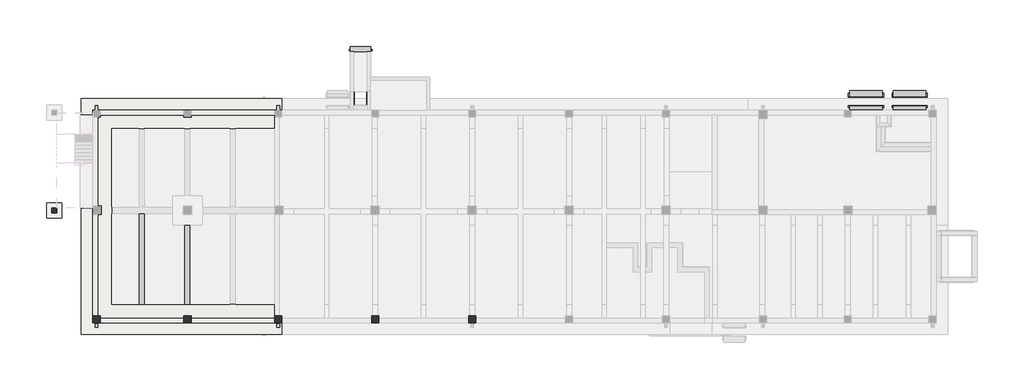
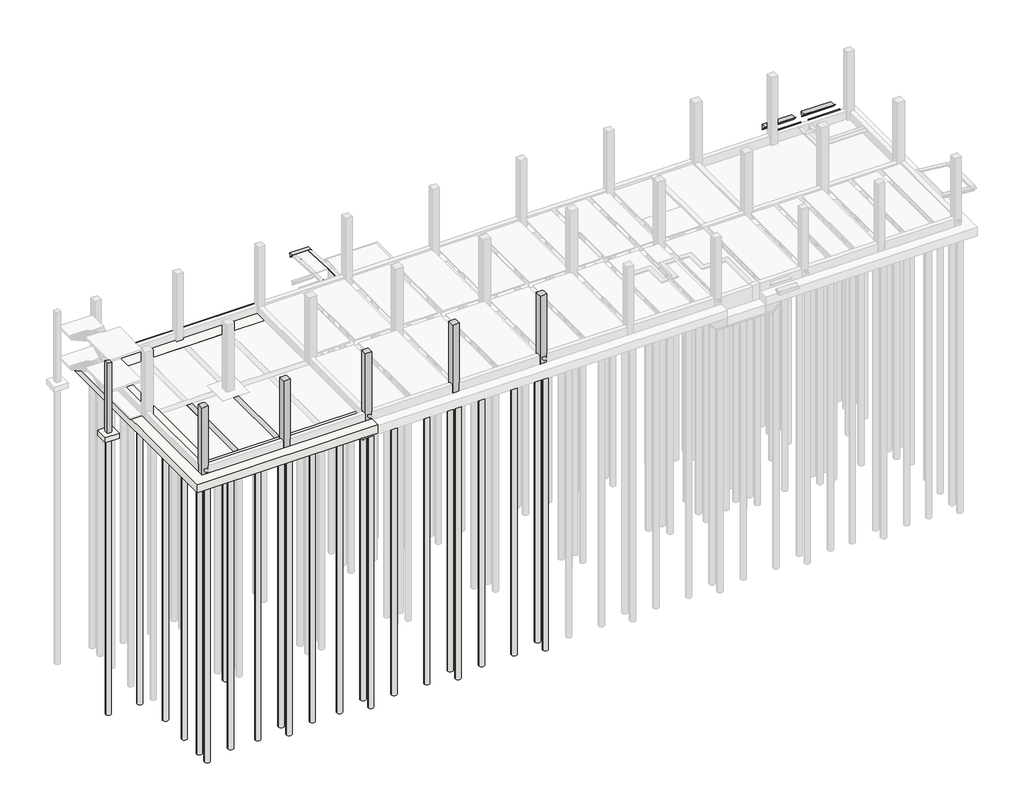
# One storey, part 3 of 7: 26 slabs, 11 proxies, 6 columns, 2 beams.
"""IFC4 building model written with IfcOpenShell, lengths in millimetres."""

from ifc_helpers import new_model, si_unit, point, frame, frame_2d, origin, place, context, project, spatial, polyline, circle_curve, trimmed, segment, composite_curve, outline, extrude, faceted_brep, element, save

model = new_model("IFC4")

# Units and contexts
model_context = context("Model", 3, world=origin())
ifc_project = project(units=[si_unit("LENGTHUNIT", "METRE", prefix="MILLI")], contexts=[model_context])

# Site, building, storey
site = spatial("IfcSite", under=ifc_project)
building = spatial("IfcBuilding", under=site)
storey = spatial("IfcBuildingStorey", under=building, Name="H.P.P", Elevation=4500.0)

# Beams
placement = place(None, origin())
element("IfcBeam", 1, ObjectType="RC Beam_Rectangular : H_SB_AR S16_TG-UG_500x700_FB1A", at=placement, inside=storey, context=model_context, shape_type="Brep", body=[
    faceted_brep([(3500.0, -15750.0, 3400.0), (4000.0, -15750.0, 3400.0), (4000.0, -15750.0, 3840.0), (4000.0, -15750.0, 3950.0), (4000.0, -15750.0, 4100.0), (3500.0, -15750.0, 4100.0), (3500.0, -15750.0, 3950.0), (3500.0, -15750.0, 3840.0), (4000.0, -8300.0, 4100.0), (3500.0, -8300.0, 4100.0), (4000.0, -8300.0, 3950.0), (4000.0, -8300.0, 3400.0), (4000.0, -8300.0, 3840.0), (3500.0, -8300.0, 3400.0), (3500.0, -8300.0, 3950.0), (3500.0, -8300.0, 3840.0)], [[[0, 1, 2, 3, 4, 5, 6, 7]], [[5, 4, 8, 9]], [[10, 8, 4, 3, 2, 1, 11, 12]], [[1, 0, 13, 11]], [[9, 14, 15, 13, 0, 7, 6, 5]], [[9, 8, 10, 12, 11, 13, 15, 14]]]),
])
element("IfcBeam", 2, ObjectType="RC Beam_Rectangular : H_SB_AR S16_TG-UG_500x700_FG1", at=placement, inside=storey, context=model_context, shape_type="Brep", body=[
    faceted_brep([(7250.0, -9250.0, 4100.0), (7750.0, -9250.0, 4100.0), (7750.0, -9250.0, 3950.0), (7750.0, -9250.0, 3840.0), (7750.0, -9250.0, 3400.0), (7250.0, -9250.0, 3400.0), (7250.0, -9250.0, 3840.0), (7250.0, -9250.0, 3950.0), (7250.0, -15750.0, 3400.0), (7750.0, -15750.0, 3400.0), (7750.0, -15750.0, 3840.0), (7750.0, -15750.0, 3950.0), (7750.0, -15750.0, 4100.0), (7250.0, -15750.0, 4100.0), (7250.0, -15750.0, 3950.0), (7250.0, -15750.0, 3840.0)], [[[0, 1, 2, 3, 4, 5, 6, 7]], [[8, 9, 10, 11, 12, 13, 14, 15]], [[1, 0, 13, 12]], [[1, 12, 11, 10, 9, 4, 3, 2]], [[5, 4, 9, 8]], [[13, 0, 7, 6, 5, 8, 15, 14]]]),
])

# Proxies
element("IfcBuildingElementProxy", 3, Name="H_SF_AR_B08_Stoop_T150_FrontEdge", ObjectType="H_SF_AR_B08_Stoop_T150_FrontEdge", at=placement, inside=storey, context=model_context, shape_type="SweptSolid", body=[
    extrude(outline(polyline([(312.0000074, 4450.0), (312.0000074, 4600.0), (662.0000074, 4600.0), (512.0000074, 4450.0), (312.0000074, 4450.0)])), frame((65750.0, 0.0, 0.0), z_axis=(1.0, 0.0, 0.0), x_axis=(0.0, 1.0, 0.0)), (0.0, 0.0, 1.0), 2700.0),
])
element("IfcBuildingElementProxy", 4, Name="H_SF_AR_B08_Stoop_T150_FrontEdge_500x300", ObjectType="H_SF_AR_B08_Stoop_T150_FrontEdge_500x300", at=placement, inside=storey, context=model_context, shape_type="Brep", body=[
    faceted_brep([(68450.0, 1900.0, 4300.0), (68450.0, 1900.0, 4600.0), (68450.0, 1600.0, 4600.0), (68450.0, 1400.0, 4600.0), (68450.0, 1700.0, 4300.0), (65750.0, 1900.0, 4300.0), (65750.0, 1700.0, 4300.0), (65750.0, 1400.0, 4600.0), (65750.0, 1600.0, 4600.0), (65750.0, 1900.0, 4600.0)], [[[0, 1, 2, 3, 4]], [[5, 6, 7, 8, 9]], [[1, 0, 5, 9]], [[3, 2, 1, 9, 8, 7]], [[4, 3, 7, 6]], [[0, 4, 6, 5]]]),
])
element("IfcBuildingElementProxy", 5, Name="H_SF_AR_S18_Lean_T50_300X300", ObjectType="H_SF_AR_S18_Lean_T50_300X300", at=placement, inside=storey, context=model_context, shape_type="SweptSolid", body=[
    extrude(outline(polyline([(1700.0, 4300.0), (1700.0, 4250.0), (1679.2893219, 4250.0), (1379.2893219, 4550.0), (1400.0, 4550.0), (1400.0, 4600.0), (1700.0, 4300.0)])), frame((65650.0, 0.0, 0.0), z_axis=(1.0, 0.0, 0.0), x_axis=(0.0, 1.0, 0.0)), (0.0, 0.0, 1.0), 2900.0),
])
element("IfcBuildingElementProxy", 6, Name="H_SF_AR_S18_Lean_T50_150X150", ObjectType="H_SF_AR_S18_Lean_T50_150X150", at=placement, inside=storey, context=model_context, shape_type="SweptSolid", body=[
    extrude(outline(polyline([(512.0000074, 4400.0), (512.0000074, 4450.0), (662.0000074, 4600.0), (662.0000074, 4550.0), (682.7106855, 4550.0), (532.7106855, 4400.0), (512.0000074, 4400.0)])), frame((65650.0, 0.0, 0.0), z_axis=(1.0, 0.0, 0.0), x_axis=(0.0, 1.0, 0.0)), (0.0, 0.0, 1.0), 2900.0),
])
element("IfcBuildingElementProxy", 7, Name="H_SF_AR_B08_Stoop_T150_FrontEdge", ObjectType="H_SF_AR_B08_Stoop_T150_FrontEdge", at=placement, inside=storey, context=model_context, shape_type="SweptSolid", body=[
    extrude(outline(polyline([(312.0000074, 4450.0), (312.0000074, 4600.0), (662.0000074, 4600.0), (512.0000074, 4450.0), (312.0000074, 4450.0)])), frame((62150.0, 0.0, 0.0), z_axis=(1.0, 0.0, 0.0), x_axis=(0.0, 1.0, 0.0)), (0.0, 0.0, 1.0), 2700.0),
])
element("IfcBuildingElementProxy", 8, Name="H_SF_AR_B08_Stoop_T150_FrontEdge_500x300", ObjectType="H_SF_AR_B08_Stoop_T150_FrontEdge_500x300", at=placement, inside=storey, context=model_context, shape_type="Brep", body=[
    faceted_brep([(64850.0, 1900.0, 4300.0), (64850.0, 1900.0, 4600.0), (64850.0, 1600.0, 4600.0), (64850.0, 1400.0, 4600.0), (64850.0, 1700.0, 4300.0), (62150.0, 1900.0, 4300.0), (62150.0, 1700.0, 4300.0), (62150.0, 1400.0, 4600.0), (62150.0, 1600.0, 4600.0), (62150.0, 1900.0, 4600.0)], [[[0, 1, 2, 3, 4]], [[5, 6, 7, 8, 9]], [[1, 0, 5, 9]], [[3, 2, 1, 9, 8, 7]], [[4, 3, 7, 6]], [[0, 4, 6, 5]]]),
])
element("IfcBuildingElementProxy", 9, Name="H_SF_AR_S18_Lean_T50_300X300", ObjectType="H_SF_AR_S18_Lean_T50_300X300", at=placement, inside=storey, context=model_context, shape_type="SweptSolid", body=[
    extrude(outline(polyline([(1700.0, 4300.0), (1700.0, 4250.0), (1679.2893219, 4250.0), (1379.2893219, 4550.0), (1400.0, 4550.0), (1400.0, 4600.0), (1700.0, 4300.0)])), frame((62050.0, 0.0, 0.0), z_axis=(1.0, 0.0, 0.0), x_axis=(0.0, 1.0, 0.0)), (0.0, 0.0, 1.0), 2900.0),
])
element("IfcBuildingElementProxy", 10, Name="H_SF_AR_S18_Lean_T50_150X150", ObjectType="H_SF_AR_S18_Lean_T50_150X150", at=placement, inside=storey, context=model_context, shape_type="SweptSolid", body=[
    extrude(outline(polyline([(512.0000074, 4400.0), (512.0000074, 4450.0), (662.0000074, 4600.0), (662.0000074, 4550.0), (682.7106855, 4550.0), (532.7106855, 4400.0), (512.0000074, 4400.0)])), frame((62050.0, 0.0, 0.0), z_axis=(1.0, 0.0, 0.0), x_axis=(0.0, 1.0, 0.0)), (0.0, 0.0, 1.0), 2900.0),
])
element("IfcBuildingElementProxy", 11, Name="H_SF_AR_B08_Ramp_T150_FrontEdge(SLOPE)", ObjectType="H_SF_AR_B08_Ramp_T150_FrontEdge(SLOPE)", at=placement, inside=storey, context=model_context, shape_type="Brep", body=[
    faceted_brep([(22638.0, 5300.0, 4179.6670362), (22638.0, 5550.0, 4179.6670362), (22638.0, 5550.0, 4349.6670362), (22638.0, 5100.0, 4379.6670362), (22638.0, 5261.0710326, 4218.5960036), (20938.0, 5550.0, 4179.6670362), (20938.0, 5300.0, 4179.6670362), (20938.0, 5261.0710326, 4218.5960036), (20938.0, 5100.0, 4379.6670362), (20938.0, 5550.0, 4349.6670362), (22338.0, 5100.0, 4379.6670362), (21238.0, 5100.0, 4379.6670362)], [[[0, 1, 2, 3, 4]], [[5, 6, 7, 8, 9]], [[1, 5, 9, 2]], [[1, 0, 6, 5]], [[0, 4, 3, 10, 11, 8, 7, 6]], [[3, 2, 9, 8, 11, 10]]]),
])
element("IfcBuildingElementProxy", 12, Name="H_SF_AR_S18_Lean_T50_200X200", ObjectType="H_SF_AR_S18_Lean_T50_200X200", at=placement, inside=storey, context=model_context, shape_type="Brep", body=[
    faceted_brep([(20838.0, 5300.0, 4179.6670362), (20838.0, 5300.0, 4129.6670362), (20838.0, 5279.2893219, 4129.6670362), (20838.0, 5184.596098, 4224.3602601), (20838.0, 5260.3575388, 4219.3094974), (22738.0, 5300.0, 4129.6670362), (22738.0, 5300.0, 4179.6670362), (22738.0, 5260.3575388, 4219.3094974), (22738.0, 5184.596098, 4224.3602601), (22738.0, 5238.2864422, 4170.6699159), (22738.0, 5279.2893219, 4129.6670362), (20938.0, 5260.3575388, 4219.3094974), (20938.0, 5261.0710326, 4218.5960036), (21088.0, 5261.0710326, 4218.5960036), (21238.0, 5100.0, 4379.6670362), (22338.0, 5100.0, 4379.6670362), (22488.0, 5261.0710326, 4218.5960036), (22638.0, 5261.0710326, 4218.5960036), (22638.0, 5260.3575388, 4219.3094974), (22638.0, 5300.0, 4179.6670362), (20938.0, 5300.0, 4179.6670362), (22638.0, 5184.596098, 4224.3602601), (22638.0, 5185.3095918, 4223.6467663), (22488.0, 5185.3095918, 4223.6467663), (22389.2669117, 5079.2893219, 4329.6670362), (22319.2206862, 5079.2893219, 4329.6670362), (21256.7793138, 5079.2893219, 4329.6670362), (21186.7330883, 5079.2893219, 4329.6670362), (21088.0, 5185.3095918, 4223.6467663), (20938.0, 5185.3095918, 4223.6467663), (20938.0, 5184.596098, 4224.3602601), (20850.0, 5184.596098, 4224.3602601), (22387.8892579, 5100.0, 4329.6670362), (22317.8430324, 5100.0, 4329.6670362), (21258.1569676, 5100.0, 4329.6670362), (21188.1107421, 5100.0, 4329.6670362)], [[[0, 1, 2, 3, 4]], [[5, 6, 7, 8, 9, 10]], [[0, 4, 11, 12, 13, 14, 15, 16, 17, 18, 7, 6, 19, 20]], [[1, 0, 20, 19, 6, 5]], [[2, 1, 5, 10]], [[2, 10, 9, 8, 21, 22, 23, 24, 25, 26, 27, 28, 29, 30, 31, 3]], [[27, 26, 25, 24, 32, 33, 34, 35]], [[15, 14, 35, 34, 33, 32]], [[8, 7, 18, 21]], [[4, 3, 31, 30, 11]], [[29, 12, 11, 30]], [[13, 28, 27, 35, 14]], [[12, 29, 28, 13]], [[17, 22, 21, 18]], [[23, 16, 15, 32, 24]], [[22, 17, 16, 23]]]),
])
element("IfcBuildingElementProxy", 13, Name="H_SF_AR_S18_Lean_T50_150X150", ObjectType="H_SF_AR_S18_Lean_T50_150X150", at=placement, inside=storey, context=model_context, shape_type="Brep", body=[
    faceted_brep([(22338.0, 1800.0, 4600.0), (22488.0, 1800.0, 4450.0), (22488.0, 1800.0, 4400.0), (22467.2893219, 1800.0, 4400.0), (22317.2893219, 1800.0, 4550.0), (22338.0, 1800.0, 4550.0), (22488.0, 550.0, 4450.0), (22338.0, 700.0, 4600.0), (22338.0, 700.0, 4550.0), (22317.2893219, 720.7106781, 4550.0), (22467.2893219, 570.7106781, 4400.0), (22488.0, 550.0, 4400.0)], [[[0, 1, 2, 3, 4, 5]], [[6, 7, 8, 9, 10, 11]], [[1, 0, 7, 6]], [[2, 1, 6, 11]], [[3, 2, 11, 10]], [[4, 3, 10, 9]], [[5, 4, 9, 8]], [[0, 5, 8, 7]]]),
    faceted_brep([(21238.0, 700.0, 4600.0), (21088.0, 550.0, 4450.0), (21088.0, 550.0, 4400.0), (21108.7106781, 570.7106781, 4400.0), (21258.7106781, 720.7106781, 4550.0), (21238.0, 700.0, 4550.0), (21088.0, 1800.0, 4450.0), (21238.0, 1800.0, 4600.0), (21238.0, 1800.0, 4550.0), (21258.7106781, 1800.0, 4550.0), (21108.7106781, 1800.0, 4400.0), (21088.0, 1800.0, 4400.0)], [[[0, 1, 2, 3, 4, 5]], [[6, 7, 8, 9, 10, 11]], [[1, 0, 7, 6]], [[2, 1, 6, 11]], [[3, 2, 11, 10]], [[4, 3, 10, 9]], [[5, 4, 9, 8]], [[0, 5, 8, 7]]]),
    faceted_brep([(22488.0, 1800.0, 4450.0), (22338.0, 1800.0, 4600.3329638), (22338.0, 1800.0, 4550.2219759), (22317.2893219, 1800.0, 4550.2219759), (22467.2893219, 1800.0, 4399.8890121), (22488.0, 1800.0, 4399.8890121), (22488.0, 5184.596098, 4224.3602601), (22389.9313644, 5079.2893219, 4329.6670362), (22388.5537105, 5100.0, 4329.6670362), (22338.6644526, 5100.0, 4379.6670362), (22338.0, 5109.9889135, 4379.6670362), (22488.0, 5238.2864422, 4170.6699159), (22467.2893219, 5238.2864422, 4170.6699159), (22317.2893219, 5100.0, 4330.2219759), (22317.8430324, 5100.0, 4329.6670362), (22319.2206862, 5079.2893219, 4329.6670362), (22338.0, 5100.0, 4330.2219759), (22338.0, 5100.0, 4379.6670362), (22389.2669117, 5079.2893219, 4329.6670362), (22387.8892579, 5100.0, 4329.6670362)], [[[0, 1, 2, 3, 4, 5]], [[1, 0, 6, 7, 8, 9, 10]], [[0, 5, 11, 6]], [[5, 4, 12, 11]], [[4, 3, 13, 14, 15, 12]], [[3, 2, 16, 13]], [[2, 1, 10, 17, 16]], [[10, 9, 17]], [[15, 18, 7, 6, 11, 12]], [[7, 18, 15, 14, 19, 8]], [[8, 19, 14, 13, 16, 17, 9]]]),
    faceted_brep([(21238.0, 1800.0, 4600.3329638), (21088.0, 1800.0, 4450.0), (21088.0, 1800.0, 4399.8890121), (21108.7106781, 1800.0, 4399.8890121), (21258.7106781, 1800.0, 4550.2219759), (21238.0, 1800.0, 4550.2219759), (21238.0, 5109.9889135, 4379.6670362), (21237.3355474, 5100.0, 4379.6670362), (21187.4462895, 5100.0, 4329.6670362), (21186.0686356, 5079.2893219, 4329.6670362), (21088.0, 5184.596098, 4224.3602601), (21088.0, 5238.2864422, 4170.6699159), (21108.7106781, 5238.2864422, 4170.6699159), (21256.7793138, 5079.2893219, 4329.6670362), (21258.1569676, 5100.0, 4329.6670362), (21258.7106781, 5100.0, 4330.2219759), (21238.0, 5100.0, 4330.2219759), (21238.0, 5100.0, 4379.6670362), (21186.7330883, 5079.2893219, 4329.6670362), (21188.1107421, 5100.0, 4329.6670362)], [[[0, 1, 2, 3, 4, 5]], [[1, 0, 6, 7, 8, 9, 10]], [[2, 1, 10, 11]], [[3, 2, 11, 12]], [[4, 3, 12, 13, 14, 15]], [[5, 4, 15, 16]], [[0, 5, 16, 17, 6]], [[7, 6, 17]], [[9, 18, 13, 12, 11, 10]], [[13, 18, 9, 8, 19, 14]], [[14, 19, 8, 7, 17, 16, 15]]]),
])

# Columns
element("IfcColumn", 14, ObjectType="RC_Column_Rectangular : H_SC_AR S15_RC Col-AG_600x600_C2", at=placement, inside=storey, context=model_context, shape_type="Brep", body=[
    faceted_brep([(30700.0, -16700.0, 4000.0), (31300.0, -16700.0, 4000.0), (31300.0, -16900.0, 4000.0), (31300.0, -17300.0, 4000.0), (30700.0, -17300.0, 4000.0), (30700.0, -16900.0, 4000.0), (30700.0, -16700.0, 4650.0), (30700.0, -16700.0, 4800.0), (30700.0, -16700.0, 10450.0), (30700.0, -16700.0, 10600.0), (30750.0000002, -16700.0, 10600.0), (31249.9999998, -16700.0, 10600.0), (31300.0, -16700.0, 10600.0), (31300.0, -16700.0, 10450.0), (31300.0, -16700.0, 4800.0), (31300.0, -16700.0, 4650.0), (31300.0, -16900.0, 10600.0), (31300.0, -17300.0, 10600.0), (31300.0, -17300.0, 9800.0), (31300.0, -17300.0, 4800.0), (30700.0, -17300.0, 10600.0), (30700.0, -17300.0, 9800.0), (30700.0, -17300.0, 4800.0), (30700.0, -16900.0, 10600.0)], [[[0, 1, 2, 3, 4, 5]], [[1, 0, 6, 7, 8, 9, 10, 11, 12, 13, 14, 15]], [[3, 2, 1, 15, 14, 13, 12, 16, 17, 18, 19]], [[4, 3, 19, 18, 17, 20, 21, 22]], [[0, 5, 4, 22, 21, 20, 23, 9, 8, 7, 6]], [[20, 17, 16, 12, 11, 10, 9, 23]]]),
])
element("IfcColumn", 15, ObjectType="RC_Column_Rectangular : H_SC_AR S15_RC Col-AG_600x600_C2", at=placement, inside=storey, context=model_context, shape_type="Brep", body=[
    faceted_brep([(22700.0, -16700.0, 4000.0), (23300.0, -16700.0, 4000.0), (23300.0, -16900.0, 4000.0), (23300.0, -17300.0, 4000.0), (22700.0, -17300.0, 4000.0), (22700.0, -16900.0, 4000.0), (22700.0, -16700.0, 4650.0), (22700.0, -16700.0, 4800.0), (22700.0, -16700.0, 10450.0), (22700.0, -16700.0, 10600.0), (23200.0, -16700.0, 10600.0), (23300.0, -16700.0, 10600.0), (23300.0, -16700.0, 10450.0), (23300.0, -16700.0, 4800.0), (23300.0, -16700.0, 4650.0), (23300.0, -16900.0, 10600.0), (23300.0, -17300.0, 10600.0), (23300.0, -17300.0, 9800.0), (23300.0, -17300.0, 4800.0), (22700.0, -17300.0, 10600.0), (22700.0, -17300.0, 9800.0), (22700.0, -17300.0, 4800.0), (22700.0, -16900.0, 10600.0)], [[[0, 1, 2, 3, 4, 5]], [[1, 0, 6, 7, 8, 9, 10, 11, 12, 13, 14]], [[3, 2, 1, 14, 13, 12, 11, 15, 16, 17, 18]], [[4, 3, 18, 17, 16, 19, 20, 21]], [[0, 5, 4, 21, 20, 19, 22, 9, 8, 7, 6]], [[19, 16, 15, 11, 10, 9, 22]]]),
])
element("IfcColumn", 16, ObjectType="RC_Column_Rectangular : H_SC_AR S15_RC Col-AG_600x600_C2", at=placement, inside=storey, context=model_context, shape_type="Brep", body=[
    faceted_brep([(14700.0, -16700.0, 4100.0), (15100.0, -16700.0, 4100.0), (15300.0, -16700.0, 4100.0), (15300.0, -17300.0, 4100.0), (14700.0, -17300.0, 4100.0), (14700.0, -16900.0, 4100.0), (14700.0, -16700.0, 4800.0), (14700.0, -16700.0, 10450.0), (14700.0, -16700.0, 10600.0), (15200.0, -16700.0, 10600.0), (15300.0, -16700.0, 10600.0), (15300.0, -16700.0, 10450.0), (15300.0, -16700.0, 4800.0), (15300.0, -16700.0, 4650.0), (15300.0, -16900.0, 10600.0), (15300.0, -17300.0, 10600.0), (15300.0, -17300.0, 9800.0), (15300.0, -17300.0, 4800.0), (14700.0, -17300.0, 10600.0), (14700.0, -17300.0, 9800.0), (14700.0, -17300.0, 4800.0), (14700.0, -16900.0, 10600.0)], [[[0, 1, 2, 3, 4, 5]], [[2, 1, 0, 6, 7, 8, 9, 10, 11, 12, 13]], [[3, 2, 13, 12, 11, 10, 14, 15, 16, 17]], [[4, 3, 17, 16, 15, 18, 19, 20]], [[0, 5, 4, 20, 19, 18, 21, 8, 7, 6]], [[18, 15, 14, 10, 9, 8, 21]]]),
])
element("IfcColumn", 17, ObjectType="RC_Column_Rectangular : H_SC_AR S15_RC Col-AG_600x600_C2", at=placement, inside=storey, context=model_context, shape_type="Brep", body=[
    faceted_brep([(7200.0, -16700.0, 4100.0), (7800.0, -16700.0, 4100.0), (7800.0, -16900.0, 4100.0), (7800.0, -17300.0, 4100.0), (7200.0, -17300.0, 4100.0), (7200.0, -16900.0, 4100.0), (7200.0, -16700.0, 10450.0), (7200.0, -16700.0, 10600.0), (7250.0, -16700.0, 10600.0), (7750.0, -16700.0, 10600.0), (7800.0, -16700.0, 10600.0), (7800.0, -16700.0, 10450.0), (7800.0, -16900.0, 10600.0), (7800.0, -17300.0, 10600.0), (7800.0, -17300.0, 9800.0), (7800.0, -17300.0, 4800.0), (7200.0, -17300.0, 10600.0), (7200.0, -17300.0, 9800.0), (7200.0, -17300.0, 4800.0), (7200.0, -16900.0, 10600.0)], [[[0, 1, 2, 3, 4, 5]], [[1, 0, 6, 7, 8, 9, 10, 11]], [[3, 2, 1, 11, 10, 12, 13, 14, 15]], [[4, 3, 15, 14, 13, 16, 17, 18]], [[0, 5, 4, 18, 17, 16, 19, 7, 6]], [[16, 13, 12, 10, 9, 8, 7, 19]]]),
])
element("IfcColumn", 18, ObjectType="RC_Column_Rectangular : H_SC_AR S15_RC Col-AG_600x600_C2", at=placement, inside=storey, context=model_context, shape_type="Brep", body=[
    faceted_brep([(-300.0, -16700.0, 4100.0), (100.0, -16700.0, 4100.0), (300.0, -16700.0, 4100.0), (300.0, -16900.0, 4100.0), (300.0, -17300.0, 4100.0), (-300.0, -17300.0, 4100.0), (-300.0, -16700.0, 4800.0), (-300.0, -16700.0, 9900.0), (-300.0, -16700.0, 10600.0), (100.0, -16700.0, 10600.0), (300.0, -16700.0, 10600.0), (300.0, -16700.0, 10450.0), (300.0, -16900.0, 10600.0), (300.0, -17300.0, 10600.0), (300.0, -17300.0, 9800.0), (300.0, -17300.0, 4800.0), (-300.0, -17300.0, 10600.0)], [[[0, 1, 2, 3, 4, 5]], [[2, 1, 0, 6, 7, 8, 9, 10, 11]], [[4, 3, 2, 11, 10, 12, 13, 14, 15]], [[5, 4, 15, 14, 13, 16]], [[0, 5, 16, 8, 7, 6]], [[16, 13, 12, 10, 9, 8]]]),
])
element("IfcColumn", 19, ObjectType="RC_Column_Rectangular : H_SC_AR S15_RC Col-AG_400x400_C3", at=placement, inside=storey, context=model_context, shape_type="Brep", body=[
    faceted_brep([(-3300.0, -7800.0, 3800.0), (-3300.0, -8200.0, 3800.0), (-3700.0, -8200.0, 3800.0), (-3700.0, -7800.0, 3800.0), (-3300.0, -7800.0, 10600.0), (-3300.0, -8200.0, 10600.0), (-3300.0, -7800.0, 4030.0), (-3300.0, -7800.0, 4630.0), (-3300.0, -7800.0, 6990.0), (-3300.0, -7800.0, 7590.0), (-3300.0, -7800.0, 9950.0), (-3300.0, -7800.0, 10550.0), (-3700.0, -8200.0, 10600.0), (-3700.0, -7800.0, 10600.0), (-3700.0, -7800.0, 10550.0), (-3700.0, -7800.0, 9950.0), (-3700.0, -7800.0, 7590.0), (-3700.0, -7800.0, 6990.0), (-3700.0, -7800.0, 4630.0), (-3700.0, -7800.0, 4030.0)], [[[0, 1, 2, 3]], [[4, 5, 1, 0, 6, 7, 8, 9, 10, 11]], [[5, 12, 2, 1]], [[12, 13, 14, 15, 16, 17, 18, 19, 3, 2]], [[13, 4, 11, 10, 9, 8, 7, 6, 0, 3, 19, 18, 17, 16, 15, 14]], [[4, 13, 12, 5]]]),
])

# Slabs
element("IfcSlab", 20, ObjectType="H_SF_AR S18_MAT_T800_WF1", at=placement, inside=storey, context=model_context, shape_type="Brep", body=[
    faceted_brep([(15299.9999999, 1249.9999999, 3300.0), (15299.9999999, -1250.0000001, 3300.0), (13799.9999999, -1250.0000001, 3300.0), (1250.0000002, -1250.0000001, 3300.0), (1250.0000002, -7700.0, 3300.0), (1250.0000002, -8300.0, 3300.0), (1250.0000002, -15750.0000001, 3300.0), (13799.9999999, -15750.0000001, 3300.0), (15299.9999999, -15750.0000001, 3300.0), (15299.9999999, -18250.0000001, 3300.0), (13799.9999999, -18250.0000001, 3300.0), (-1250.0, -18250.0000001, 3300.0), (-1250.0, 1249.9999999, 3300.0), (13799.9999999, 1249.9999999, 3300.0), (15299.9999999, 1249.9999999, 4100.0), (-1250.0, 1249.9999999, 4100.0), (-1250.0, -18250.0000001, 4100.0), (15299.9999999, -18250.0000001, 4100.0), (15299.9999999, -15750.0000001, 4100.0), (15200.0208108, -15750.0000001, 4100.0), (14975.0010428, -15750.0000001, 4100.0), (11500.0, -15750.0000001, 4100.0), (11000.0, -15750.0000001, 4100.0), (7750.0, -15750.0000001, 4100.0), (7250.0, -15750.0000001, 4100.0), (4000.0, -15750.0000001, 4100.0), (3500.0, -15750.0000001, 4100.0), (1250.0000002, -15750.0000001, 4100.0), (1250.0000002, -8300.0, 4100.0), (1250.0000002, -7700.0, 4100.0), (1250.0000002, -1250.0000001, 4100.0), (3500.0, -1250.0000001, 4100.0), (4000.0, -1250.0000001, 4100.0), (7250.0, -1250.0000001, 4100.0), (7750.0, -1250.0000001, 4100.0), (11000.0, -1250.0000001, 4100.0), (11500.0, -1250.0000001, 4100.0), (14975.0013677, -1250.0000001, 4100.0), (15200.0274333, -1250.0000001, 4100.0), (15299.9999999, -1250.0000001, 4100.0), (15299.9999999, -18250.0000001, 4000.0), (15299.9999999, 1249.9999999, 4000.0), (15299.9999999, -15750.0000001, 4000.0), (15299.9999999, -1250.0000001, 4000.0)], [[[0, 1, 2, 3, 4, 5, 6, 7, 8, 9, 10, 11, 12, 13]], [[14, 15, 16, 17, 18, 19, 20, 21, 22, 23, 24, 25, 26, 27, 28, 29, 30, 31, 32, 33, 34, 35, 36, 37, 38, 39]], [[11, 10, 9, 40, 17, 16]], [[12, 11, 16, 15]], [[0, 13, 12, 15, 14, 41]], [[6, 5, 4, 3, 30, 29, 28, 27]], [[8, 7, 6, 27, 26, 25, 24, 23, 22, 21, 20, 19, 18, 42]], [[3, 2, 1, 43, 39, 38, 37, 36, 35, 34, 33, 32, 31, 30]], [[1, 0, 41, 14, 39, 43]], [[9, 8, 42, 18, 17, 40]]]),
])
element("IfcSlab", 21, ObjectType="H_SF_AR_S18_Lean_T50", at=placement, inside=storey, context=model_context, shape_type="SweptSolid", body=[
    extrude(outline(polyline([(3390.0, -1360.0000001), (3390.0, -7590.0), (1360.0000002, -7590.0), (1360.0000002, -1360.0000001), (3390.0, -1360.0000001)])), frame((0.0, 0.0, 3790.0), z_axis=(0.0, 0.0, 1.0), x_axis=(1.0, 0.0, 0.0)), (0.0, 0.0, 1.0), 50.0),
    extrude(outline(polyline([(3390.0, -8410.0), (3390.0, -15640.0000001), (1360.0000002, -15640.0000001), (1360.0000002, -8410.0), (3390.0, -8410.0)])), frame((0.0, 0.0, 3790.0), z_axis=(0.0, 0.0, 1.0), x_axis=(1.0, 0.0, 0.0)), (0.0, 0.0, 1.0), 50.0),
    extrude(outline(polyline([(6250.0, -8410.0), (6250.0, -9250.0), (7140.0, -9250.0), (7140.0, -15640.0000001), (4110.0, -15640.0000001), (4110.0, -8410.0), (6250.0, -8410.0)])), frame((0.0, 0.0, 3790.0), z_axis=(0.0, 0.0, 1.0), x_axis=(1.0, 0.0, 0.0)), (0.0, 0.0, 1.0), 50.0),
    extrude(outline(polyline([(6250.0, -7590.0), (4110.0, -7590.0), (4110.0, -1360.0000001), (7140.0, -1360.0000001), (7140.0, -6750.0), (6250.0, -6750.0), (6250.0, -7590.0)])), frame((0.0, 0.0, 3790.0), z_axis=(0.0, 0.0, 1.0), x_axis=(1.0, 0.0, 0.0)), (0.0, 0.0, 1.0), 50.0),
    extrude(outline(polyline([(8750.0, -8410.0), (10890.0, -8410.0), (10890.0, -15640.0000001), (7860.0, -15640.0000001), (7860.0, -9250.0), (8750.0, -9250.0), (8750.0, -8410.0)])), frame((0.0, 0.0, 3790.0), z_axis=(0.0, 0.0, 1.0), x_axis=(1.0, 0.0, 0.0)), (0.0, 0.0, 1.0), 50.0),
    extrude(outline(polyline([(8750.0, -7590.0), (8750.0, -6750.0), (7860.0, -6750.0), (7860.0, -1360.0000001), (10890.0, -1360.0000001), (10890.0, -7590.0), (8750.0, -7590.0)])), frame((0.0, 0.0, 3790.0), z_axis=(0.0, 0.0, 1.0), x_axis=(1.0, 0.0, 0.0)), (0.0, 0.0, 1.0), 50.0),
    extrude(outline(polyline([(13800.0000001, -8410.0), (13800.0000001, -9250.0), (14590.0, -9250.0), (14590.0, -15640.0000001), (11610.0, -15640.0000001), (11610.0, -8410.0), (13800.0000001, -8410.0)])), frame((0.0, 0.0, 3790.0), z_axis=(0.0, 0.0, 1.0), x_axis=(1.0, 0.0, 0.0)), (0.0, 0.0, 1.0), 50.0),
    extrude(outline(polyline([(13800.0000001, -7590.0), (11610.0, -7590.0), (11610.0, -1360.0000001), (14590.0, -1360.0000001), (14590.0, -6750.0), (13800.0000001, -6750.0), (13800.0000001, -7590.0)])), frame((0.0, 0.0, 3790.0), z_axis=(0.0, 0.0, 1.0), x_axis=(1.0, 0.0, 0.0)), (0.0, 0.0, 1.0), 50.0),
])
element("IfcSlab", 22, ObjectType="Foundation Rectangular (Non-Pile) : H_SF_AR S18_Ret Fdn_1250x1250xT500_F2", at=placement, inside=storey, context=model_context, shape_type="SweptSolid", body=[
    extrude(outline(polyline([(-2875.0, -7375.0), (-2875.0, -8625.0), (-4125.0, -8625.0), (-4125.0, -7375.0), (-2875.0, -7375.0)])), frame((0.0, 0.0, 3300.0), z_axis=(0.0, 0.0, 1.0), x_axis=(1.0, 0.0, 0.0)), (0.0, 0.0, 1.0), 500.0),
])
element("IfcSlab", 23, ObjectType="PILE : H_FL_AR S19_Pile_D500_L26.9", at=placement, inside=storey, context=model_context, shape_type="SweptSolid", body=[
    extrude(outline(composite_curve([segment(trimmed(circle_curve(frame_2d((-3500.0, -8000.0)), 250.0), [point((-3750.0, -8000.0))], [point((-3250.0, -8000.0))], False, "CARTESIAN"), True, "CONTINUOUS"), segment(trimmed(circle_curve(frame_2d((-3500.0, -8000.0)), 250.0), [point((-3250.0, -8000.0))], [point((-3750.0, -8000.0))], False, "CARTESIAN"), True, "CONTINUOUS")], self_intersect=False)), frame((0.0, 0.0, -23500.0), z_axis=(0.0, 0.0, 1.0), x_axis=(1.0, 0.0, 0.0)), (0.0, 0.0, 1.0), 26750.0),
])
element("IfcSlab", 24, ObjectType="PILE : H_FL_AR S19_Pile_D500_L26.9", at=placement, inside=storey, context=model_context, shape_type="SweptSolid", body=[
    extrude(outline(composite_curve([segment(trimmed(circle_curve(frame_2d((-625.0000004, -8000.0)), 250.0), [point((-875.0000004, -8000.0))], [point((-375.0000004, -8000.0))], False, "CARTESIAN"), True, "CONTINUOUS"), segment(trimmed(circle_curve(frame_2d((-625.0000004, -8000.0)), 250.0), [point((-375.0000004, -8000.0))], [point((-875.0000004, -8000.0))], False, "CARTESIAN"), True, "CONTINUOUS")], self_intersect=False)), frame((0.0, 0.0, -23500.0), z_axis=(0.0, 0.0, 1.0), x_axis=(1.0, 0.0, 0.0)), (0.0, 0.0, 1.0), 26750.0),
])
element("IfcSlab", 25, ObjectType="PILE : H_FL_AR S19_Pile_D500_L26.9", at=placement, inside=storey, context=model_context, shape_type="SweptSolid", body=[
    extrude(outline(composite_curve([segment(trimmed(circle_curve(frame_2d((0.0, -11000.0000003)), 250.0), [point((-250.0, -11000.0000003))], [point((250.0, -11000.0000003))], False, "CARTESIAN"), True, "CONTINUOUS"), segment(trimmed(circle_curve(frame_2d((0.0, -11000.0000003)), 250.0), [point((250.0, -11000.0000003))], [point((-250.0, -11000.0000003))], False, "CARTESIAN"), True, "CONTINUOUS")], self_intersect=False)), frame((0.0, 0.0, -23500.0), z_axis=(0.0, 0.0, 1.0), x_axis=(1.0, 0.0, 0.0)), (0.0, 0.0, 1.0), 26750.0),
])
element("IfcSlab", 26, ObjectType="PILE : H_FL_AR S19_Pile_D500_L26.9", at=placement, inside=storey, context=model_context, shape_type="SweptSolid", body=[
    extrude(outline(composite_curve([segment(trimmed(circle_curve(frame_2d((0.0, -14000.0000004)), 250.0), [point((-250.0, -14000.0000004))], [point((250.0, -14000.0000004))], False, "CARTESIAN"), True, "CONTINUOUS"), segment(trimmed(circle_curve(frame_2d((0.0, -14000.0000004)), 250.0), [point((250.0, -14000.0000004))], [point((-250.0, -14000.0000004))], False, "CARTESIAN"), True, "CONTINUOUS")], self_intersect=False)), frame((0.0, 0.0, -23500.0), z_axis=(0.0, 0.0, 1.0), x_axis=(1.0, 0.0, 0.0)), (0.0, 0.0, 1.0), 26750.0),
])
element("IfcSlab", 27, ObjectType="PILE : H_FL_AR S19_Pile_D500_L26.7", at=placement, inside=storey, context=model_context, shape_type="SweptSolid", body=[
    extrude(outline(composite_curve([segment(trimmed(circle_curve(frame_2d((6875.0000004, -8624.9999999)), 250.0), [point((6625.0000004, -8624.9999999))], [point((7125.0000004, -8624.9999999))], False, "CARTESIAN"), True, "CONTINUOUS"), segment(trimmed(circle_curve(frame_2d((6875.0000004, -8624.9999999)), 250.0), [point((7125.0000004, -8624.9999999))], [point((6625.0000004, -8624.9999999))], False, "CARTESIAN"), True, "CONTINUOUS")], self_intersect=False)), frame((0.0, 0.0, -23500.0), z_axis=(0.0, 0.0, 1.0), x_axis=(1.0, 0.0, 0.0)), (0.0, 0.0, 1.0), 26550.0),
])
element("IfcSlab", 28, ObjectType="PILE : H_FL_AR S19_Pile_D500_L26.9", at=placement, inside=storey, context=model_context, shape_type="SweptSolid", body=[
    extrude(outline(composite_curve([segment(trimmed(circle_curve(frame_2d((0.0, -16375.0000004)), 250.0), [point((-250.0, -16375.0000004))], [point((250.0, -16375.0000004))], False, "CARTESIAN"), True, "CONTINUOUS"), segment(trimmed(circle_curve(frame_2d((0.0, -16375.0000004)), 250.0), [point((250.0, -16375.0000004))], [point((-250.0, -16375.0000004))], False, "CARTESIAN"), True, "CONTINUOUS")], self_intersect=False)), frame((0.0, 0.0, -23500.0), z_axis=(0.0, 0.0, 1.0), x_axis=(1.0, 0.0, 0.0)), (0.0, 0.0, 1.0), 26750.0),
])
element("IfcSlab", 29, ObjectType="PILE : H_FL_AR S19_Pile_D500_L26.9", at=placement, inside=storey, context=model_context, shape_type="SweptSolid", body=[
    extrude(outline(composite_curve([segment(trimmed(circle_curve(frame_2d((0.0, -17625.0)), 250.0), [point((-250.0, -17625.0))], [point((250.0, -17625.0))], False, "CARTESIAN"), True, "CONTINUOUS"), segment(trimmed(circle_curve(frame_2d((0.0, -17625.0)), 250.0), [point((250.0, -17625.0))], [point((-250.0, -17625.0))], False, "CARTESIAN"), True, "CONTINUOUS")], self_intersect=False)), frame((0.0, 0.0, -23500.0), z_axis=(0.0, 0.0, 1.0), x_axis=(1.0, 0.0, 0.0)), (0.0, 0.0, 1.0), 26750.0),
])
element("IfcSlab", 30, ObjectType="PILE : H_FL_AR S19_Pile_D500_L26.9", at=placement, inside=storey, context=model_context, shape_type="SweptSolid", body=[
    extrude(outline(composite_curve([segment(trimmed(circle_curve(frame_2d((2506.7380833, -17000.0)), 250.0), [point((2256.7380833, -17000.0))], [point((2756.7380833, -17000.0))], False, "CARTESIAN"), True, "CONTINUOUS"), segment(trimmed(circle_curve(frame_2d((2506.7380833, -17000.0)), 250.0), [point((2756.7380833, -17000.0))], [point((2256.7380833, -17000.0))], False, "CARTESIAN"), True, "CONTINUOUS")], self_intersect=False)), frame((0.0, 0.0, -23500.0), z_axis=(0.0, 0.0, 1.0), x_axis=(1.0, 0.0, 0.0)), (0.0, 0.0, 1.0), 26750.0),
])
element("IfcSlab", 31, ObjectType="PILE : H_FL_AR S19_Pile_D500_L26.9", at=placement, inside=storey, context=model_context, shape_type="SweptSolid", body=[
    extrude(outline(composite_curve([segment(trimmed(circle_curve(frame_2d((5000.0000002, -17000.0)), 250.0), [point((4750.0000002, -17000.0))], [point((5250.0000002, -17000.0))], False, "CARTESIAN"), True, "CONTINUOUS"), segment(trimmed(circle_curve(frame_2d((5000.0000002, -17000.0)), 250.0), [point((5250.0000002, -17000.0))], [point((4750.0000002, -17000.0))], False, "CARTESIAN"), True, "CONTINUOUS")], self_intersect=False)), frame((0.0, 0.0, -23500.0), z_axis=(0.0, 0.0, 1.0), x_axis=(1.0, 0.0, 0.0)), (0.0, 0.0, 1.0), 26750.0),
])
element("IfcSlab", 32, ObjectType="PILE : H_FL_AR S19_Pile_D500_L26.9", at=placement, inside=storey, context=model_context, shape_type="SweptSolid", body=[
    extrude(outline(composite_curve([segment(trimmed(circle_curve(frame_2d((7500.0, -16375.0000002)), 250.0), [point((7250.0, -16375.0000002))], [point((7750.0, -16375.0000002))], False, "CARTESIAN"), True, "CONTINUOUS"), segment(trimmed(circle_curve(frame_2d((7500.0, -16375.0000002)), 250.0), [point((7750.0, -16375.0000002))], [point((7250.0, -16375.0000002))], False, "CARTESIAN"), True, "CONTINUOUS")], self_intersect=False)), frame((0.0, 0.0, -23500.0), z_axis=(0.0, 0.0, 1.0), x_axis=(1.0, 0.0, 0.0)), (0.0, 0.0, 1.0), 26750.0),
])
element("IfcSlab", 33, ObjectType="PILE : H_FL_AR S19_Pile_D500_L26.9", at=placement, inside=storey, context=model_context, shape_type="SweptSolid", body=[
    extrude(outline(composite_curve([segment(trimmed(circle_curve(frame_2d((7500.0, -17624.9999998)), 250.0), [point((7250.0, -17624.9999998))], [point((7750.0, -17624.9999998))], False, "CARTESIAN"), True, "CONTINUOUS"), segment(trimmed(circle_curve(frame_2d((7500.0, -17624.9999998)), 250.0), [point((7750.0, -17624.9999998))], [point((7250.0, -17624.9999998))], False, "CARTESIAN"), True, "CONTINUOUS")], self_intersect=False)), frame((0.0, 0.0, -23500.0), z_axis=(0.0, 0.0, 1.0), x_axis=(1.0, 0.0, 0.0)), (0.0, 0.0, 1.0), 26750.0),
])
element("IfcSlab", 34, ObjectType="PILE : H_FL_AR S19_Pile_D500_L26.9", at=placement, inside=storey, context=model_context, shape_type="SweptSolid", body=[
    extrude(outline(composite_curve([segment(trimmed(circle_curve(frame_2d((10000.0000006, -17000.0)), 250.0), [point((9750.0000006, -17000.0))], [point((10250.0000006, -17000.0))], False, "CARTESIAN"), True, "CONTINUOUS"), segment(trimmed(circle_curve(frame_2d((10000.0000006, -17000.0)), 250.0), [point((10250.0000006, -17000.0))], [point((9750.0000006, -17000.0))], False, "CARTESIAN"), True, "CONTINUOUS")], self_intersect=False)), frame((0.0, 0.0, -23500.0), z_axis=(0.0, 0.0, 1.0), x_axis=(1.0, 0.0, 0.0)), (0.0, 0.0, 1.0), 26750.0),
])
element("IfcSlab", 35, ObjectType="PILE : H_FL_AR S19_Pile_D500_L26.9", at=placement, inside=storey, context=model_context, shape_type="SweptSolid", body=[
    extrude(outline(composite_curve([segment(trimmed(circle_curve(frame_2d((12500.0000009, -17000.0)), 250.0), [point((12250.0000009, -17000.0))], [point((12750.0000009, -17000.0))], False, "CARTESIAN"), True, "CONTINUOUS"), segment(trimmed(circle_curve(frame_2d((12500.0000009, -17000.0)), 250.0), [point((12750.0000009, -17000.0))], [point((12250.0000009, -17000.0))], False, "CARTESIAN"), True, "CONTINUOUS")], self_intersect=False)), frame((0.0, 0.0, -23500.0), z_axis=(0.0, 0.0, 1.0), x_axis=(1.0, 0.0, 0.0)), (0.0, 0.0, 1.0), 26750.0),
])
element("IfcSlab", 36, ObjectType="PILE : H_FL_AR S19_Pile_D500_L26.8", at=placement, inside=storey, context=model_context, shape_type="SweptSolid", body=[
    extrude(outline(composite_curve([segment(trimmed(circle_curve(frame_2d((14999.9999999, -16375.0000004)), 250.0), [point((15249.9999999, -16375.0000004))], [point((14749.9999999, -16375.0000004))], False, "CARTESIAN"), True, "CONTINUOUS"), segment(trimmed(circle_curve(frame_2d((14999.9999999, -16375.0000004)), 250.0), [point((14749.9999999, -16375.0000004))], [point((15249.9999999, -16375.0000004))], False, "CARTESIAN"), True, "CONTINUOUS")], self_intersect=False)), frame((0.0, 0.0, 3200.0), z_axis=(0.0, 0.0, 1.0), x_axis=(1.0, 0.0, 0.0)), (0.0, 0.0, 1.0), 100.0),
    extrude(outline(composite_curve([segment(trimmed(circle_curve(frame_2d((14999.9999999, -16375.0000004)), 250.0), [point((14749.9999999, -16375.0000004))], [point((15249.9999999, -16375.0000004))], False, "CARTESIAN"), True, "CONTINUOUS"), segment(trimmed(circle_curve(frame_2d((14999.9999999, -16375.0000004)), 250.0), [point((15249.9999999, -16375.0000004))], [point((14749.9999999, -16375.0000004))], False, "CARTESIAN"), True, "CONTINUOUS")], self_intersect=False)), frame((0.0, 0.0, -23500.0), z_axis=(0.0, 0.0, 1.0), x_axis=(1.0, 0.0, 0.0)), (0.0, 0.0, 1.0), 26650.0),
])
element("IfcSlab", 37, ObjectType="PILE : H_FL_AR S19_Pile_D500_L26.8", at=placement, inside=storey, context=model_context, shape_type="SweptSolid", body=[
    extrude(outline(composite_curve([segment(trimmed(circle_curve(frame_2d((14999.9999999, -17625.0)), 250.0), [point((15249.9999999, -17625.0))], [point((14749.9999999, -17625.0))], False, "CARTESIAN"), True, "CONTINUOUS"), segment(trimmed(circle_curve(frame_2d((14999.9999999, -17625.0)), 250.0), [point((14749.9999999, -17625.0))], [point((15249.9999999, -17625.0))], False, "CARTESIAN"), True, "CONTINUOUS")], self_intersect=False)), frame((0.0, 0.0, 3200.0), z_axis=(0.0, 0.0, 1.0), x_axis=(1.0, 0.0, 0.0)), (0.0, 0.0, 1.0), 100.0),
    extrude(outline(composite_curve([segment(trimmed(circle_curve(frame_2d((14999.9999999, -17625.0)), 250.0), [point((14749.9999999, -17625.0))], [point((15249.9999999, -17625.0))], False, "CARTESIAN"), True, "CONTINUOUS"), segment(trimmed(circle_curve(frame_2d((14999.9999999, -17625.0)), 250.0), [point((15249.9999999, -17625.0))], [point((14749.9999999, -17625.0))], False, "CARTESIAN"), True, "CONTINUOUS")], self_intersect=False)), frame((0.0, 0.0, -23500.0), z_axis=(0.0, 0.0, 1.0), x_axis=(1.0, 0.0, 0.0)), (0.0, 0.0, 1.0), 26650.0),
])
element("IfcSlab", 38, ObjectType="PILE : H_FL_AR S19_Pile_D500_L26.8", at=placement, inside=storey, context=model_context, shape_type="SweptSolid", body=[
    extrude(outline(composite_curve([segment(trimmed(circle_curve(frame_2d((17500.0000012, -17000.0)), 250.0), [point((17250.0000012, -17000.0))], [point((17750.0000012, -17000.0))], False, "CARTESIAN"), True, "CONTINUOUS"), segment(trimmed(circle_curve(frame_2d((17500.0000012, -17000.0)), 250.0), [point((17750.0000012, -17000.0))], [point((17250.0000012, -17000.0))], False, "CARTESIAN"), True, "CONTINUOUS")], self_intersect=False)), frame((0.0, 0.0, -23500.0), z_axis=(0.0, 0.0, 1.0), x_axis=(1.0, 0.0, 0.0)), (0.0, 0.0, 1.0), 26650.0),
])
element("IfcSlab", 39, ObjectType="PILE : H_FL_AR S19_Pile_D500_L26.8", at=placement, inside=storey, context=model_context, shape_type="SweptSolid", body=[
    extrude(outline(composite_curve([segment(trimmed(circle_curve(frame_2d((20500.0000002, -17000.0)), 250.0), [point((20250.0000002, -17000.0))], [point((20750.0000002, -17000.0))], False, "CARTESIAN"), True, "CONTINUOUS"), segment(trimmed(circle_curve(frame_2d((20500.0000002, -17000.0)), 250.0), [point((20750.0000002, -17000.0))], [point((20250.0000002, -17000.0))], False, "CARTESIAN"), True, "CONTINUOUS")], self_intersect=False)), frame((0.0, 0.0, -23500.0), z_axis=(0.0, 0.0, 1.0), x_axis=(1.0, 0.0, 0.0)), (0.0, 0.0, 1.0), 26650.0),
])
element("IfcSlab", 40, ObjectType="PILE : H_FL_AR S19_Pile_D500_L26.8", at=placement, inside=storey, context=model_context, shape_type="SweptSolid", body=[
    extrude(outline(composite_curve([segment(trimmed(circle_curve(frame_2d((23000.0, -16375.0)), 250.0), [point((22750.0, -16375.0))], [point((23250.0, -16375.0))], False, "CARTESIAN"), True, "CONTINUOUS"), segment(trimmed(circle_curve(frame_2d((23000.0, -16375.0)), 250.0), [point((23250.0, -16375.0))], [point((22750.0, -16375.0))], False, "CARTESIAN"), True, "CONTINUOUS")], self_intersect=False)), frame((0.0, 0.0, -23500.0), z_axis=(0.0, 0.0, 1.0), x_axis=(1.0, 0.0, 0.0)), (0.0, 0.0, 1.0), 26650.0),
])
element("IfcSlab", 41, ObjectType="PILE : H_FL_AR S19_Pile_D500_L26.8", at=placement, inside=storey, context=model_context, shape_type="SweptSolid", body=[
    extrude(outline(composite_curve([segment(trimmed(circle_curve(frame_2d((23000.0, -17624.9999996)), 250.0), [point((22750.0, -17624.9999996))], [point((23250.0, -17624.9999996))], False, "CARTESIAN"), True, "CONTINUOUS"), segment(trimmed(circle_curve(frame_2d((23000.0, -17624.9999996)), 250.0), [point((23250.0, -17624.9999996))], [point((22750.0, -17624.9999996))], False, "CARTESIAN"), True, "CONTINUOUS")], self_intersect=False)), frame((0.0, 0.0, -23500.0), z_axis=(0.0, 0.0, 1.0), x_axis=(1.0, 0.0, 0.0)), (0.0, 0.0, 1.0), 26650.0),
])
element("IfcSlab", 42, ObjectType="PILE : H_FL_AR S19_Pile_D500_L26.8", at=placement, inside=storey, context=model_context, shape_type="SweptSolid", body=[
    extrude(outline(composite_curve([segment(trimmed(circle_curve(frame_2d((25500.0000012, -17000.0)), 250.0), [point((25250.0000012, -17000.0))], [point((25750.0000012, -17000.0))], False, "CARTESIAN"), True, "CONTINUOUS"), segment(trimmed(circle_curve(frame_2d((25500.0000012, -17000.0)), 250.0), [point((25750.0000012, -17000.0))], [point((25250.0000012, -17000.0))], False, "CARTESIAN"), True, "CONTINUOUS")], self_intersect=False)), frame((0.0, 0.0, -23500.0), z_axis=(0.0, 0.0, 1.0), x_axis=(1.0, 0.0, 0.0)), (0.0, 0.0, 1.0), 26650.0),
])
element("IfcSlab", 43, ObjectType="PILE : H_FL_AR S19_Pile_D500_L26.8", at=placement, inside=storey, context=model_context, shape_type="SweptSolid", body=[
    extrude(outline(composite_curve([segment(trimmed(circle_curve(frame_2d((28500.0000003, -17000.0)), 250.0), [point((28250.0000003, -17000.0))], [point((28750.0000003, -17000.0))], False, "CARTESIAN"), True, "CONTINUOUS"), segment(trimmed(circle_curve(frame_2d((28500.0000003, -17000.0)), 250.0), [point((28750.0000003, -17000.0))], [point((28250.0000003, -17000.0))], False, "CARTESIAN"), True, "CONTINUOUS")], self_intersect=False)), frame((0.0, 0.0, -23500.0), z_axis=(0.0, 0.0, 1.0), x_axis=(1.0, 0.0, 0.0)), (0.0, 0.0, 1.0), 26650.0),
])
element("IfcSlab", 44, ObjectType="PILE : H_FL_AR S19_Pile_D500_L26.8", at=placement, inside=storey, context=model_context, shape_type="SweptSolid", body=[
    extrude(outline(composite_curve([segment(trimmed(circle_curve(frame_2d((31000.0, -16375.0000004)), 250.0), [point((30750.0, -16375.0000004))], [point((31250.0, -16375.0000004))], False, "CARTESIAN"), True, "CONTINUOUS"), segment(trimmed(circle_curve(frame_2d((31000.0, -16375.0000004)), 250.0), [point((31250.0, -16375.0000004))], [point((30750.0, -16375.0000004))], False, "CARTESIAN"), True, "CONTINUOUS")], self_intersect=False)), frame((0.0, 0.0, -23500.0), z_axis=(0.0, 0.0, 1.0), x_axis=(1.0, 0.0, 0.0)), (0.0, 0.0, 1.0), 26650.0),
])
element("IfcSlab", 45, ObjectType="PILE : H_FL_AR S19_Pile_D500_L26.8", at=placement, inside=storey, context=model_context, shape_type="SweptSolid", body=[
    extrude(outline(composite_curve([segment(trimmed(circle_curve(frame_2d((31000.0, -17625.0)), 250.0), [point((30750.0, -17625.0))], [point((31250.0, -17625.0))], False, "CARTESIAN"), True, "CONTINUOUS"), segment(trimmed(circle_curve(frame_2d((31000.0, -17625.0)), 250.0), [point((31250.0, -17625.0))], [point((30750.0, -17625.0))], False, "CARTESIAN"), True, "CONTINUOUS")], self_intersect=False)), frame((0.0, 0.0, -23500.0), z_axis=(0.0, 0.0, 1.0), x_axis=(1.0, 0.0, 0.0)), (0.0, 0.0, 1.0), 26650.0),
])

save(model, "model.ifc")

# Revit data of these elements
# Type "RC Beam_Rectangular : H_SB_AR S16_TG-UG_500x700_FB1A"
#   Type Comments = "CV-UG"
#   중앙부 하부근 = ""
#   중앙부 상부근 = ""
#   중앙부 보조근 = ""
#   중앙부 늑근 = ""
#   외단부 하부근 = ""
#   외단부 상부근 = ""
#   외단부 보조근 = ""
#   외단부 늑근 = ""
#   부호 = "TG3"
#   내단부 하부근 = ""
#   내단부 상부근 = ""
#   내단부 보조근 = ""
#   내단부 늑근 = ""
#   ALL 하부근 = "3-D20"
#   ALL 상부근 = "3-D20"
#   ALL 보조근 = ""
#   ALL 늑근 = "2-D10 @120"
#   H_Rebar Ratio = 0.14
#   Width = 500 mm
#   Height = 700 mm
#   Length [instance default] = 1524 mm
#   b = 500 mm
#   h = 700 mm
#   hec_material3 [instance default] = none
#   hec_material2 [instance default] = none
#   hec_material1 [instance default] = none
#   Structural Material [instance default] = none
#   Assembly Code = ""
# Type "RC Beam_Rectangular : H_SB_AR S16_TG-UG_500x700_FG1"
#   Type Comments = "CV-UG"
#   중앙부 하부근 = ""
#   중앙부 상부근 = ""
#   중앙부 보조근 = ""
#   중앙부 늑근 = ""
#   외단부 하부근 = ""
#   외단부 상부근 = ""
#   외단부 보조근 = ""
#   외단부 늑근 = ""
#   부호 = "TG3"
#   내단부 하부근 = ""
#   내단부 상부근 = ""
#   내단부 보조근 = ""
#   내단부 늑근 = ""
#   ALL 하부근 = "3-D20"
#   ALL 상부근 = "3-D20"
#   ALL 보조근 = ""
#   ALL 늑근 = "2-D10 @120"
#   H_Rebar Ratio = 0.14
#   Width = 500 mm
#   Height = 700 mm
#   Length [instance default] = 1524 mm
#   b = 500 mm
#   h = 700 mm
#   hec_material3 [instance default] = none
#   hec_material2 [instance default] = none
#   hec_material1 [instance default] = none
#   Structural Material [instance default] = none
#   Assembly Code = ""
# Type "H_SF_AR_B08_Stoop_T150_FrontEdge"
#   Type Comments = "CV-UG"
#   H_Rebar Ratio = 0.12
# Type "H_SF_AR_B08_Stoop_T150_FrontEdge_500x300"
#   Type Comments = "CV-UG"
#   H_Rebar Ratio = 0.12
# Type "H_SF_AR_S18_Lean_T50_300X300"
#   Type Comments = "Lean"
# Type "H_SF_AR_S18_Lean_T50_150X150"
#   Type Comments = "Lean"
# Type "H_SF_AR_B08_Ramp_T150_FrontEdge(SLOPE)"
#   Type Comments = "CV-UG"
#   H_Rebar Ratio = 0.12
# Type "H_SF_AR_S18_Lean_T50_200X200"
#   Type Comments = "Lean"
# Type "RC_Column_Rectangular : H_SC_AR S15_RC Col-AG_600x600_C2"
#   Type Comments = "CV-AG"
#   H_Rebar Ratio = 0.3
#   Width = 600 mm
#   Depth = 600 mm
#   hec_material3 [instance default] = none
#   hec_material2 [instance default] = none
#   hec_material1 [instance default] = none
#   Structural Material [instance default] = none
#   Description = (empty or 0)
# Type "RC_Column_Rectangular : H_SC_AR S15_RC Col-AG_400x400_C3"
#   Type Comments = "CV-AG"
#   H_Rebar Ratio = 0.3
#   Width = 400 mm
#   Depth = 400 mm
#   hec_material3 [instance default] = none
#   hec_material2 [instance default] = none
#   hec_material1 [instance default] = none
#   Structural Material [instance default] = none
#   Description = (empty or 0)
# Type "H_SF_AR S18_MAT_T800_WF1"
#   Type Comments = "CV-UG"
#   H_Rebar Ratio = 0.12
#   Layers, outside or top first: 800 mm "Concrete_f'c=28MPa(Cylender)" (function 1)
# Type "H_SF_AR_S18_Lean_T50"
#   Type Comments = "Lean"
#   Layers, outside or top first: 50 mm "Concrete_f'c=14MPa(Cylender)" (function 1)
# Type "Foundation Rectangular (Non-Pile) : H_SF_AR S18_Ret Fdn_1250x1250xT500_F2"
#   Top bar = "D25@300"
#   Description = "UG Shallow Foundation"
#   Bottom bar = "D20@300"
#   Width = 1250 mm
#   Length = 1250 mm
#   Foundation Thickness = 500 mm
#   Structural Material [instance default] = none
#   Assembly Code = ""
# Type "PILE : H_FL_AR S19_Pile_D500_L26.9"
#   Type Comments = "Pile"
#   Assembly Code = "A1020120"
#   반지름 = 250 mm
#   최소 내포 = 150 mm
#   Diameter = 500 mm
#   Depth = 26750 mm
#   Structural Material [instance default] = none
# Type "PILE : H_FL_AR S19_Pile_D500_L26.7"
#   Type Comments = "Pile"
#   Assembly Code = "A1020120"
#   반지름 = 250 mm
#   최소 내포 = 150 mm
#   Diameter = 500 mm
#   Depth = 26550 mm
#   Structural Material [instance default] = none
# Type "PILE : H_FL_AR S19_Pile_D500_L26.8"
#   Type Comments = "Pile"
#   Assembly Code = "A1020120"
#   반지름 = 250 mm
#   최소 내포 = 150 mm
#   Diameter = 500 mm
#   Depth = 26650 mm
#   Structural Material [instance default] = none
# Element 1 (IfcBeam, "RC Beam_Rectangular : H_SB_AR S16_TG-UG_500x700_FB1A")
#   Comments = ""
#   hec_material3 = none
#   hec_material2 = none
#   hec_material1 = none
#   Structural Material = Concrete_f'c=28MPa(Cylender)
#   Phase Created = New Construction
#   Materials on its faces: "Concrete_f'c=28MPa(Cylender)"
# Element 2 (IfcBeam, "RC Beam_Rectangular : H_SB_AR S16_TG-UG_500x700_FG1")
#   Comments = ""
#   hec_material3 = none
#   hec_material2 = none
#   hec_material1 = none
#   Structural Material = Concrete_f'c=28MPa(Cylender)
#   Phase Created = New Construction
#   Materials on its faces: "Concrete_f'c=28MPa(Cylender)"
# Elements 3, 7 (IfcBuildingElementProxy, "H_SF_AR_B08_Stoop_T150_FrontEdge")
#   Phase Created = New Construction
#   Materials on its faces: "Concrete_f'c=28MPa(Cylender)"
# Elements 4, 8 (IfcBuildingElementProxy, "H_SF_AR_B08_Stoop_T150_FrontEdge_500x300")
#   built-in parameter 1012827 = 0.328084 (stored number, unit not read)
#   Phase Created = New Construction
#   Materials on its faces: "Concrete_f'c=28MPa(Cylender)"
# Elements 5, 9 (IfcBuildingElementProxy, "H_SF_AR_S18_Lean_T50_300X300")
#   built-in parameter 1012827 = 0.984252 (stored number, unit not read)
#   built-in parameter 1012825 = -0.984252 (stored number, unit not read)
#   Phase Created = New Construction
#   Materials on its faces: "Concrete_f'c=14MPa(Cylender)"
# Elements 6, 10, 13 (IfcBuildingElementProxy, "H_SF_AR_S18_Lean_T50_150X150")
#   built-in parameter 1012827 = 0.492126 (stored number, unit not read)
#   built-in parameter 1012825 = -0.492126 (stored number, unit not read)
#   Phase Created = New Construction
#   Materials on its faces: "Concrete_f'c=14MPa(Cylender)"
# Element 11 (IfcBuildingElementProxy, "H_SF_AR_B08_Ramp_T150_FrontEdge(SLOPE)")
#   built-in parameter 1012827 = 0.0984252 (stored number, unit not read)
#   Phase Created = New Construction
#   Materials on its faces: "Concrete_f'c=28MPa(Cylender)"
# Element 12 (IfcBuildingElementProxy, "H_SF_AR_S18_Lean_T50_200X200")
#   built-in parameter 1012827 = 0.656168 (stored number, unit not read)
#   built-in parameter 1012825 = -0.656168 (stored number, unit not read)
#   Phase Created = New Construction
#   Materials on its faces: "Concrete_f'c=14MPa(Cylender)"
# Elements 14, 15, 16, 17, 18 (IfcColumn, "RC_Column_Rectangular : H_SC_AR S15_RC Col-AG_600x600_C2")
#   Comments = ""
#   hec_material3 = none
#   hec_material2 = none
#   hec_material1 = none
#   Structural Material = Concrete_f'c=28MPa(Cylender)
#   Phase Created = New Construction
#   Materials on its faces: "Concrete_f'c=28MPa(Cylender)"
# Element 19 (IfcColumn, "RC_Column_Rectangular : H_SC_AR S15_RC Col-AG_400x400_C3")
#   Comments = ""
#   hec_material3 = none
#   hec_material2 = none
#   hec_material1 = none
#   Structural Material = Concrete_f'c=28MPa(Cylender)
#   Phase Created = New Construction
#   Materials on its faces: "Concrete_f'c=28MPa(Cylender)"
# Element 20 (IfcSlab, "H_SF_AR S18_MAT_T800_WF1")
#   Comments = ""
#   Height Offset From Level = -400 mm
#   built-in parameter 1001954 = 1
#   Phase Created = New Construction
#   Materials on its faces: "Concrete_f'c=28MPa(Cylender)"
# Element 21 (IfcSlab, "H_SF_AR_S18_Lean_T50")
#   Comments = ""
#   Height Offset From Level = -660 mm
#   built-in parameter 1001954 = 1
#   Phase Created = New Construction
#   Materials on its faces: "Concrete_f'c=14MPa(Cylender)"
# Element 22 (IfcSlab, "Foundation Rectangular (Non-Pile) : H_SF_AR S18_Ret Fdn_1250x1250xT500_F2")
#   Comments = ""
#   Structural Material = none
#   Phase Created = New Construction
# Elements 23, 24, 25, 26, 28, 29, 30, 31, 32, 33, 34, 35 (IfcSlab, "PILE : H_FL_AR S19_Pile_D500_L26.9")
#   Structural Material = Concrete_f'c=28MPa(Cylender)
#   Phase Created = New Construction
#   Materials on its faces: "Concrete_f'c=28MPa(Cylender)"
# Element 27 (IfcSlab, "PILE : H_FL_AR S19_Pile_D500_L26.7")
#   Structural Material = Concrete_f'c=28MPa(Cylender)
#   Phase Created = New Construction
#   Materials on its faces: "Concrete_f'c=28MPa(Cylender)"
# Elements 36, 37, 38, 39, 40, 41, 42, 43, 44, 45 (IfcSlab, "PILE : H_FL_AR S19_Pile_D500_L26.8")
#   Structural Material = Concrete_f'c=28MPa(Cylender)
#   Phase Created = New Construction
#   Materials on its faces: "Concrete_f'c=28MPa(Cylender)"
# Materials
#   "Concrete_f'c=28MPa(Cylender)": class "Concrete", colour RGB 176 176 176, transparency 0, Description = "Reinf. Conc.", Cost = 0, Image = Concrete.Cast-In-Place.Flat.Polished.Grey.jpg
#   "Concrete_f'c=14MPa(Cylender)": class "Concrete", colour RGB 177 177 177, transparency 0, Description = "Reinf. Conc.", Cost = 0
